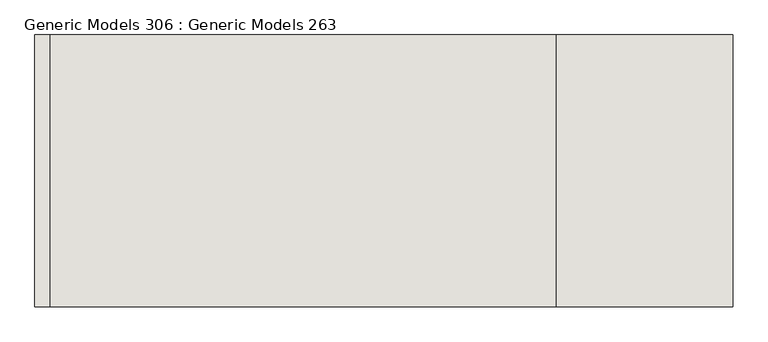
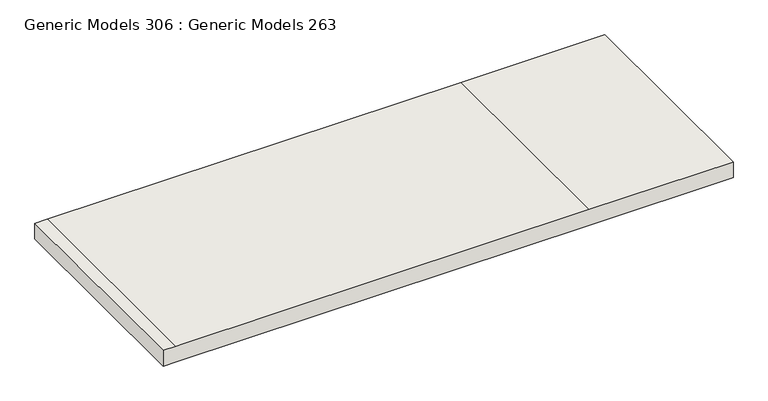
"""IFC4 building model written with IfcOpenShell, lengths in millimetres: wall geometry, Generic Models 306 : Generic Models 263."""

from ifc_helpers import new_model, si_unit, point, frame, frame_2d, origin, place, context, project, spatial, polyline, circle_curve, trimmed, segment, composite_curve, outline, extrude, source, transform, mapped, element, save


def generic_models_306_generic_models_263_110f4e42(model_context):
    return source(origin(), model_context, "Body", "SweptSolid", [
        extrude(outline(composite_curve([segment(polyline([(-304.9836851, 64122.5797726), (-304.9836851, 63653.8340403), (-914.0337686, 63653.8340403), (-914.0337686, 64148.9956464)]), True, "CONTINUOUS"), segment(trimmed(circle_curve(frame_2d((-219607.3320282, 71742.5797726)), 218825.0927648), [point((-914.0337686, 64148.9956464))], [point((-914.5836851, 79351.9848532))], True, "CARTESIAN"), True, "CONTINUOUS"), segment(polyline([(-914.5836851, 79351.9848532), (-914.5836851, 84681.146689), (-304.9836851, 84681.146689), (-304.9836851, 79362.5797726)]), True, "CONTINUOUS"), segment(trimmed(circle_curve(frame_2d((-219607.3320282, 71742.5797726)), 219434.6927648), [point((-304.9836851, 79362.5797726))], [point((-304.9836851, 64122.5797726))], False, "CARTESIAN"), True, "CONTINUOUS")], self_intersect=False)), frame((0.0, -3202.6200333, 0.0), z_axis=(0.0, 1.0, 0.0), x_axis=(0.0, 0.0, 1.0)), (0.0, 0.0, 1.0), 8183.6367002),
    ])


if __name__ == "__main__":
    model = new_model("IFC4")
    model_context = context("Model", 3, world=origin())
    ifc_project = project(units=[si_unit("LENGTHUNIT", "METRE", prefix="MILLI")], contexts=[model_context])
    site = spatial("IfcSite", under=ifc_project)
    building = spatial("IfcBuilding", under=site)
    placement = place(None, origin())
    generic_models_306_generic_models_263_shape = generic_models_306_generic_models_263_110f4e42(model_context)
    element("IfcWall", 1, ObjectType="Generic Models 306 : Generic Models 263", at=placement, inside=building, context=model_context, shape_type="MappedRepresentation", body=[
        mapped(generic_models_306_generic_models_263_shape, transform((0.0, 0.0, 0.0), x_axis=(1.0, 0.0, 0.0), y_axis=(0.0, 1.0, 0.0), z_axis=(0.0, 0.0, 1.0))),
    ])
    save(model, "model.ifc")

# Revit data of these elements
# Element 1 (IfcWall, "Generic Models 306 : Generic Models 263")
#   Materials on its faces: "EXISTING GRADE"
# Materials
#   "EXISTING GRADE": class "Miscellaneous", colour RGB 128 97 77, transparency 0, Cost = 0
